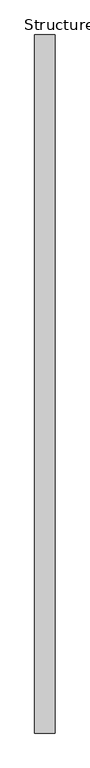
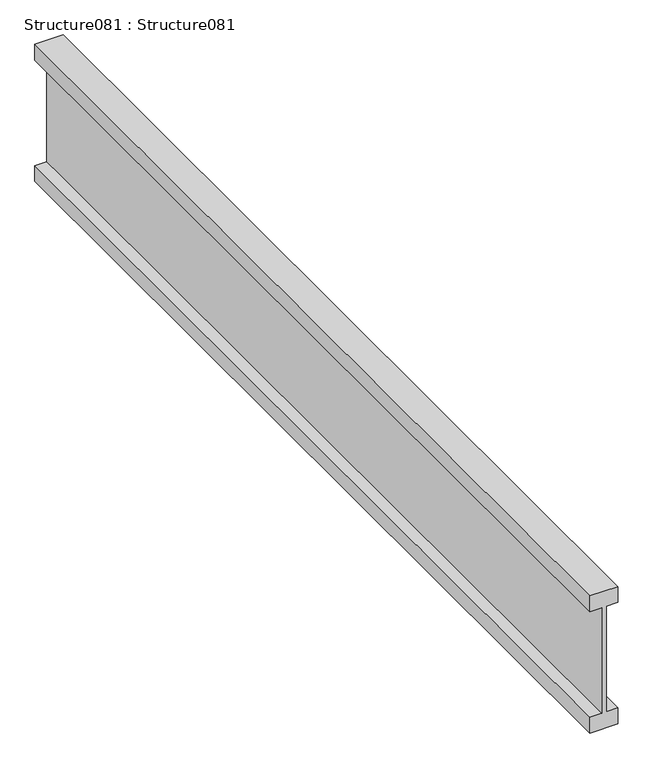
"""IFC4 building model written with IfcOpenShell, lengths in millimetres: proxy geometry, Structure081 : Structure081."""

from ifc_helpers import new_model, si_unit, frame, origin, place, context, project, spatial, polyline, outline, extrude, source, transform, mapped, element, save


def structure081_structure081_a3d9cc12(model_context):
    return source(origin(), model_context, "Body", "SweptSolid", [
        extrude(outline(polyline([(36420.171, -3218.0168586), (36420.171, -3193.4106086), (36188.396, -3193.4106086), (36188.396, -3218.0168586), (36153.471, -3218.0168586), (36153.471, -3159.2793586), (36188.396, -3159.2793586), (36188.396, -3183.8856086), (36420.171, -3183.8856086), (36420.171, -3159.2793586), (36455.096, -3159.2793586), (36455.096, -3218.0168586), (36420.171, -3218.0168586)])), frame((0.0, 998.1570053, 0.0), z_axis=(0.0, 1.0, 0.0), x_axis=(0.0, 0.0, 1.0)), (0.0, 0.0, 1.0), 2000.0),
    ])


if __name__ == "__main__":
    model = new_model("IFC4")
    model_context = context("Model", 3, world=origin())
    ifc_project = project(units=[si_unit("LENGTHUNIT", "METRE", prefix="MILLI")], contexts=[model_context])
    site = spatial("IfcSite", under=ifc_project)
    building = spatial("IfcBuilding", under=site)
    placement = place(None, origin())
    structure081_structure081_shape = structure081_structure081_a3d9cc12(model_context)
    element("IfcBuildingElementProxy", 1, Name="Structure081 : Structure081", ObjectType="Structure081 : Structure081", at=placement, inside=building, context=model_context, shape_type="MappedRepresentation", body=[
        mapped(structure081_structure081_shape, transform((0.0, 0.0, 0.0), x_axis=(1.0, 0.0, 0.0), y_axis=(0.0, 1.0, 0.0), z_axis=(0.0, 0.0, 1.0))),
    ])
    save(model, "model.ifc")

# Revit data of these elements
# Type "Structure081 : Structure081"
#   NameOverride = "Structure081"
# Element 1 (IfcBuildingElementProxy, "Structure081 : Structure081")
#   Materials on its faces: "WOOD FRAMING (SEE STRUCT DWGS)"
# Materials
#   "WOOD FRAMING (SEE STRUCT DWGS)": class "Unassigned", colour RGB 224 188 168, transparency 0, Cost = 0
